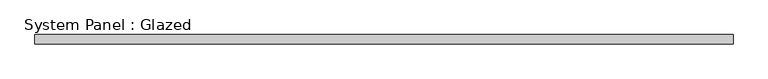
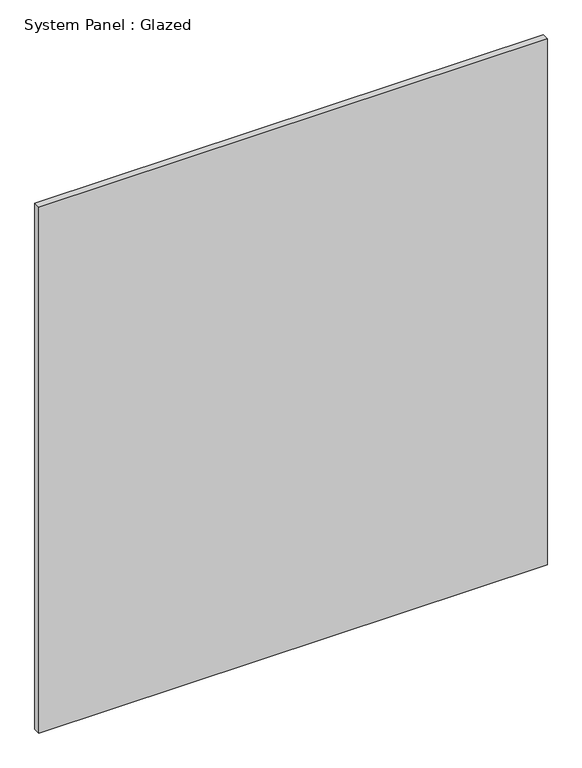
"""IFC4 building model written with IfcOpenShell, lengths in millimetres: plate geometry, System Panel : Glazed."""

from ifc_helpers import new_model, si_unit, origin, origin_with_axes, place, context, project, spatial, polyline, outline, extrude, source, transform, mapped, element, save


def system_panel_glazed_1aac6df6(model_context):
    return source(origin(), model_context, "Body", "SweptSolid", [
        extrude(outline(polyline([(915.0000002, 24.5), (-915.0000002, 24.5), (-915.0000002, 49.5), (915.0000002, 49.5), (915.0000002, 24.5)])), origin_with_axes(), (0.0, 0.0, 1.0), 2000.0),
    ])


if __name__ == "__main__":
    model = new_model("IFC4")
    model_context = context("Model", 3, world=origin())
    ifc_project = project(units=[si_unit("LENGTHUNIT", "METRE", prefix="MILLI")], contexts=[model_context])
    site = spatial("IfcSite", under=ifc_project)
    building = spatial("IfcBuilding", under=site)
    placement = place(None, origin())
    system_panel_glazed_shape = system_panel_glazed_1aac6df6(model_context)
    element("IfcPlate", 1, ObjectType="System Panel : Glazed", at=placement, inside=building, context=model_context, shape_type="MappedRepresentation", body=[
        mapped(system_panel_glazed_shape, transform((0.0, 0.0, 0.0), x_axis=(1.0, 0.0, 0.0), y_axis=(0.0, 1.0, 0.0), z_axis=(0.0, 0.0, 1.0))),
    ])
    save(model, "model.ifc")

# Revit data of these elements
# Element 1 (IfcPlate, "System Panel : Glazed")
#   Materials on its faces: "Glass"
# Materials
#   "Glass": class "Glass", colour RGB 218 227 224, transparency 0.85, Description = "Soda Lime Glass", Cost = 0
